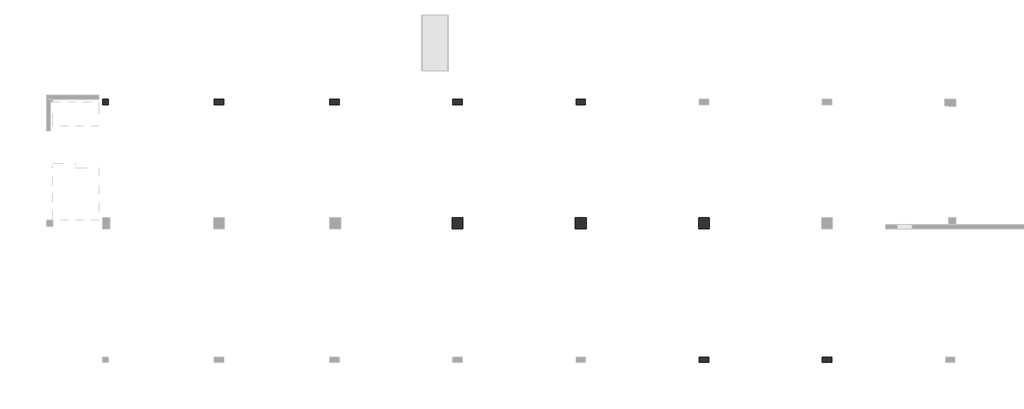
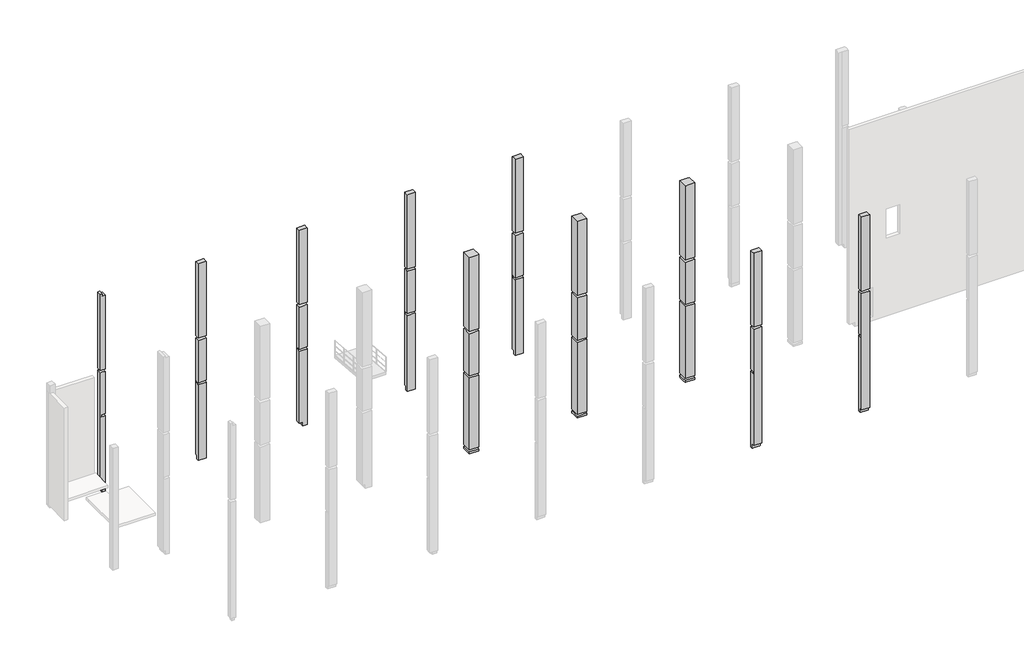
# One storey, part 2 of 3: 10 columns.
"""IFC4 building model written with IfcOpenShell, lengths in millimetres."""

from ifc_helpers import new_model, si_unit, origin, place, context, project, spatial, faceted_brep, element, save

model = new_model("IFC4")

# Units and contexts
model_context = context("Model", 3, world=origin())
ifc_project = project(units=[si_unit("LENGTHUNIT", "METRE", prefix="MILLI")], contexts=[model_context])

# Site, building, storey
site = spatial("IfcSite", under=ifc_project)
building = spatial("IfcBuilding", under=site)
storey = spatial("IfcBuildingStorey", under=building, Name="G.L", Elevation=-150.0381366)

# Columns
placement = place(None, origin())
element("IfcColumn", 1, ObjectType="RC_Column_Rectangular : H_SC_AR_S15_AG_W700xL700_C1", at=placement, inside=storey, context=model_context, shape_type="Brep", body=[
    faceted_brep([(23350.0, 9849.5208589, -150.0381366), (23350.0, 9749.5208589, -150.0381366), (23350.0, 9149.5208589, -150.0381366), (22750.0, 9149.5208589, -150.0381366), (22650.0, 9149.5208589, -150.0381366), (22650.0, 9849.5208589, -150.0381366), (22750.0, 9849.5208589, -150.0381366), (23250.0, 9849.5208589, -150.0381366), (23350.0, 9149.5208589, -0.0381366), (23350.0, 9749.5208589, -0.0381366), (23350.0, 9849.5208589, -0.0381366), (23250.0, 9849.5208589, -0.0381366), (22750.0, 9849.5208589, -0.0381366), (22650.0, 9849.5208589, -0.0381366), (22650.0, 9149.5208589, -0.0381366), (22750.0, 9149.5208589, -0.0381366), (23250.0, 9149.5208589, -0.0381366)], [[[0, 1, 2, 3, 4, 5, 6, 7]], [[8, 9, 10, 11, 12, 13, 14, 15, 16]], [[2, 1, 0, 10, 9, 8]], [[4, 3, 2, 8, 16, 15, 14]], [[5, 4, 14, 13]], [[0, 7, 6, 5, 13, 12, 11, 10]]]),
    faceted_brep([(23350.0, 9149.5208589, 9449.9618634), (23350.0, 9849.5208589, 9449.9618634), (23350.0, 9849.5208589, 15259.9618634), (23350.0, 9724.5208589, 15259.9618634), (23350.0, 9274.5208589, 15259.9618634), (23350.0, 9149.5208589, 15259.9618634), (22650.0, 9149.5208589, 9449.9618634), (23225.0, 9149.5208589, 15259.9618634), (22775.0, 9149.5208589, 15259.9618634), (22650.0, 9149.5208589, 15259.9618634), (22650.0, 9849.5208589, 9449.9618634), (22650.0, 9274.5208589, 15259.9618634), (22650.0, 9724.5208589, 15259.9618634), (22650.0, 9849.5208589, 15259.9618634), (22775.0, 9849.5208589, 15259.9618634), (23225.0, 9849.5208589, 15259.9618634)], [[[0, 1, 2, 3, 4, 5]], [[6, 0, 5, 7, 8, 9]], [[10, 6, 9, 11, 12, 13]], [[1, 10, 13, 14, 15, 2]], [[1, 0, 6, 10]], [[5, 4, 3, 2, 15, 14, 13, 12, 11, 9, 8, 7]]]),
    faceted_brep([(23350.0, 9849.5208589, 149.9618634), (23350.0, 9149.5208589, 149.9618634), (22650.0, 9149.5208589, 149.9618634), (22650.0, 9849.5208589, 149.9618634), (23350.0, 9149.5208589, 5799.9618634), (23350.0, 9199.5208589, 5799.9618634), (23350.0, 9799.5208589, 5799.9618634), (23350.0, 9849.5208589, 5799.9618634), (23250.0, 9849.5208589, 5799.9618634), (22750.0, 9849.5208589, 5799.9618634), (22650.0, 9849.5208589, 5799.9618634), (22650.0, 9799.5208589, 5799.9618634), (22650.0, 9199.5208589, 5799.9618634), (22650.0, 9149.5208589, 5799.9618634), (22750.0, 9149.5208589, 5799.9618634), (23250.0, 9149.5208589, 5799.9618634)], [[[0, 1, 2, 3]], [[4, 5, 6, 7, 8, 9, 10, 11, 12, 13, 14, 15]], [[1, 0, 7, 6, 5, 4]], [[2, 1, 4, 15, 14, 13]], [[3, 2, 13, 12, 11, 10]], [[0, 3, 10, 9, 8, 7]]]),
    faceted_brep([(23350.0, 9849.5208589, 5949.9618634), (23350.0, 9149.5208589, 5949.9618634), (22650.0, 9149.5208589, 5949.9618634), (22650.0, 9849.5208589, 5949.9618634), (23350.0, 9149.5208589, 9269.9618634), (23350.0, 9199.5208589, 9269.9618634), (23350.0, 9799.5208589, 9269.9618634), (23350.0, 9849.5208589, 9269.9618634), (23250.0, 9849.5208589, 9269.9618634), (22750.0, 9849.5208589, 9269.9618634), (22650.0, 9849.5208589, 9269.9618634), (22650.0, 9799.5208589, 9269.9618634), (22650.0, 9199.5208589, 9269.9618634), (22650.0, 9149.5208589, 9269.9618634), (22750.0, 9149.5208589, 9269.9618634), (23250.0, 9149.5208589, 9269.9618634)], [[[0, 1, 2, 3]], [[4, 5, 6, 7, 8, 9, 10, 11, 12, 13, 14, 15]], [[1, 0, 7, 6, 5, 4]], [[2, 1, 4, 15, 14, 13]], [[3, 2, 13, 12, 11, 10]], [[0, 3, 10, 9, 8, 7]]]),
])
element("IfcColumn", 2, ObjectType="RC_Column_Rectangular : H_SC_AR_S15_AG_W700xL700_C1", at=placement, inside=storey, context=model_context, shape_type="Brep", body=[
    faceted_brep([(31350.0, 9849.5208589, -150.0381366), (31350.0, 9749.5208589, -150.0381366), (31350.0, 9149.5208589, -150.0381366), (31250.0, 9149.5208589, -150.0381366), (30650.0, 9149.5208589, -150.0381366), (30650.0, 9749.5208589, -150.0381366), (30650.0, 9849.5208589, -150.0381366), (30750.0, 9849.5208589, -150.0381366), (31250.0, 9849.5208589, -150.0381366), (31350.0, 9149.5208589, -0.0381366), (31350.0, 9749.5208589, -0.0381366), (31350.0, 9849.5208589, -0.0381366), (31250.0, 9849.5208589, -0.0381366), (30750.0, 9849.5208589, -0.0381366), (30650.0, 9849.5208589, -0.0381366), (30650.0, 9749.5208589, -0.0381366), (30650.0, 9149.5208589, -0.0381366), (30750.0, 9149.5208589, -0.0381366), (31250.0, 9149.5208589, -0.0381366)], [[[0, 1, 2, 3, 4, 5, 6, 7, 8]], [[9, 10, 11, 12, 13, 14, 15, 16, 17, 18]], [[2, 1, 0, 11, 10, 9]], [[4, 3, 2, 9, 18, 17, 16]], [[6, 5, 4, 16, 15, 14]], [[0, 8, 7, 6, 14, 13, 12, 11]]]),
    faceted_brep([(31350.0, 9149.5208589, 9449.9618634), (31350.0, 9849.5208589, 9449.9618634), (31350.0, 9849.5208589, 15259.9618634), (31350.0, 9724.5208589, 15259.9618634), (31350.0, 9274.5208589, 15259.9618634), (31350.0, 9149.5208589, 15259.9618634), (30650.0, 9149.5208589, 9449.9618634), (31225.0, 9149.5208589, 15259.9618634), (30775.0, 9149.5208589, 15259.9618634), (30650.0, 9149.5208589, 15259.9618634), (30650.0, 9849.5208589, 9449.9618634), (30650.0, 9274.5208589, 15259.9618634), (30650.0, 9724.5208589, 15259.9618634), (30650.0, 9849.5208589, 15259.9618634), (30775.0, 9849.5208589, 15259.9618634), (31225.0, 9849.5208589, 15259.9618634)], [[[0, 1, 2, 3, 4, 5]], [[6, 0, 5, 7, 8, 9]], [[10, 6, 9, 11, 12, 13]], [[1, 10, 13, 14, 15, 2]], [[1, 0, 6, 10]], [[5, 4, 3, 2, 15, 14, 13, 12, 11, 9, 8, 7]]]),
    faceted_brep([(31350.0, 9849.5208589, 149.9618634), (31350.0, 9149.5208589, 149.9618634), (30650.0, 9149.5208589, 149.9618634), (30650.0, 9849.5208589, 149.9618634), (31350.0, 9149.5208589, 5799.9618634), (31350.0, 9199.5208589, 5799.9618634), (31350.0, 9799.5208589, 5799.9618634), (31350.0, 9849.5208589, 5799.9618634), (31250.0, 9849.5208589, 5799.9618634), (30750.0, 9849.5208589, 5799.9618634), (30650.0, 9849.5208589, 5799.9618634), (30650.0, 9799.5208589, 5799.9618634), (30650.0, 9199.5208589, 5799.9618634), (30650.0, 9149.5208589, 5799.9618634), (30750.0, 9149.5208589, 5799.9618634), (31250.0, 9149.5208589, 5799.9618634)], [[[0, 1, 2, 3]], [[4, 5, 6, 7, 8, 9, 10, 11, 12, 13, 14, 15]], [[1, 0, 7, 6, 5, 4]], [[2, 1, 4, 15, 14, 13]], [[3, 2, 13, 12, 11, 10]], [[0, 3, 10, 9, 8, 7]]]),
    faceted_brep([(31350.0, 9849.5208589, 5949.9618634), (31350.0, 9149.5208589, 5949.9618634), (30650.0, 9149.5208589, 5949.9618634), (30650.0, 9849.5208589, 5949.9618634), (31350.0, 9149.5208589, 9269.9618634), (31350.0, 9199.5208589, 9269.9618634), (31350.0, 9799.5208589, 9269.9618634), (31350.0, 9849.5208589, 9269.9618634), (31250.0, 9849.5208589, 9269.9618634), (30750.0, 9849.5208589, 9269.9618634), (30650.0, 9849.5208589, 9269.9618634), (30650.0, 9799.5208589, 9269.9618634), (30650.0, 9199.5208589, 9269.9618634), (30650.0, 9149.5208589, 9269.9618634), (30750.0, 9149.5208589, 9269.9618634), (31250.0, 9149.5208589, 9269.9618634)], [[[0, 1, 2, 3]], [[4, 5, 6, 7, 8, 9, 10, 11, 12, 13, 14, 15]], [[1, 0, 7, 6, 5, 4]], [[2, 1, 4, 15, 14, 13]], [[3, 2, 13, 12, 11, 10]], [[0, 3, 10, 9, 8, 7]]]),
])
element("IfcColumn", 3, ObjectType="RC_Column_Rectangular : H_SC_AR_S15_AG_W700xL700_C1", at=placement, inside=storey, context=model_context, shape_type="Brep", body=[
    faceted_brep([(39350.0, 9849.5208589, -150.0381366), (39350.0, 9749.5208589, -150.0381366), (39350.0, 9149.5208589, -150.0381366), (38750.0, 9149.5208589, -150.0381366), (38749.6109568, 9149.5208589, -150.0381366), (38650.0, 9149.5208589, -150.0381366), (38650.0, 9499.9097478, -150.0381366), (38650.0, 9749.5208589, -150.0381366), (38650.0, 9849.5208589, -150.0381366), (38750.0, 9849.5208589, -150.0381366), (39250.0, 9849.5208589, -150.0381366), (39350.0, 9149.5208589, -0.0381366), (39350.0, 9749.5208589, -0.0381366), (39350.0, 9849.5208589, -0.0381366), (39250.0, 9849.5208589, -0.0381366), (38750.0, 9849.5208589, -0.0381366), (38650.0, 9849.5208589, -0.0381366), (38650.0, 9749.5208589, -0.0381366), (38650.0, 9499.9097478, -0.0381366), (38650.0, 9149.5208589, -0.0381366)], [[[0, 1, 2, 3, 4, 5, 6, 7, 8, 9, 10]], [[11, 12, 13, 14, 15, 16, 17, 18, 19]], [[2, 1, 0, 13, 12, 11]], [[5, 4, 3, 2, 11, 19]], [[8, 7, 6, 5, 19, 18, 17, 16]], [[0, 10, 9, 8, 16, 15, 14, 13]]]),
    faceted_brep([(39350.0, 9149.5208589, 9449.9618634), (39350.0, 9849.5208589, 9449.9618634), (39350.0, 9849.5208589, 15259.9618634), (39350.0, 9149.5208589, 15259.9618634), (38650.0, 9149.5208589, 9449.9618634), (38650.0, 9149.5208589, 15259.9618634), (38650.0, 9849.5208589, 9449.9618634), (38650.0, 9849.5208589, 15259.9618634), (38775.0, 9849.5208589, 15259.9618634), (39225.0, 9849.5208589, 15259.9618634)], [[[0, 1, 2, 3]], [[4, 0, 3, 5]], [[6, 4, 5, 7]], [[1, 6, 7, 8, 9, 2]], [[1, 0, 4, 6]], [[3, 2, 9, 8, 7, 5]]]),
    faceted_brep([(39350.0, 9849.5208589, 149.9618634), (39350.0, 9149.5208589, 149.9618634), (38650.0, 9149.5208589, 149.9618634), (38650.0, 9849.5208589, 149.9618634), (39350.0, 9149.5208589, 5799.9618634), (39350.0, 9199.5208589, 5799.9618634), (39350.0, 9799.5208589, 5799.9618634), (39350.0, 9849.5208589, 5799.9618634), (39250.0, 9849.5208589, 5799.9618634), (38750.0, 9849.5208589, 5799.9618634), (38650.0, 9849.5208589, 5799.9618634), (38650.0, 9799.5208589, 5799.9618634), (38650.0, 9199.5208589, 5799.9618634), (38650.0, 9149.5208589, 5799.9618634)], [[[0, 1, 2, 3]], [[4, 5, 6, 7, 8, 9, 10, 11, 12, 13]], [[1, 0, 7, 6, 5, 4]], [[2, 1, 4, 13]], [[3, 2, 13, 12, 11, 10]], [[0, 3, 10, 9, 8, 7]]]),
    faceted_brep([(39350.0, 9849.5208589, 5949.9618634), (39350.0, 9149.5208589, 5949.9618634), (38650.0, 9149.5208589, 5949.9618634), (38650.0, 9849.5208589, 5949.9618634), (39350.0, 9149.5208589, 9269.9618634), (39350.0, 9199.5208589, 9269.9618634), (39350.0, 9799.5208589, 9269.9618634), (39350.0, 9849.5208589, 9269.9618634), (39250.0, 9849.5208589, 9269.9618634), (38750.0, 9849.5208589, 9269.9618634), (38650.0, 9849.5208589, 9269.9618634), (38650.0, 9799.5208589, 9269.9618634), (38650.0, 9199.5208589, 9269.9618634), (38650.0, 9149.5208589, 9269.9618634)], [[[0, 1, 2, 3]], [[4, 5, 6, 7, 8, 9, 10, 11, 12, 13]], [[1, 0, 7, 6, 5, 4]], [[2, 1, 4, 13]], [[3, 2, 13, 12, 11, 10]], [[0, 3, 10, 9, 8, 7]]]),
])
element("IfcColumn", 4, ObjectType="RC_Column_Rectangular : H_SC_AR_S15_AG_W600xL600_C2", at=placement, inside=storey, context=model_context, shape_type="Brep", body=[
    faceted_brep([(300.0, 17199.5208589, -150.0381366), (100.0, 17199.5208589, -150.0381366), (100.0, 17399.5208589, -150.0381366), (300.0, 17399.5208589, -150.0381366), (300.0, 17499.5208589, 5799.9618634), (0.0, 17499.5208589, 5799.9618634), (0.0, 17199.5208589, 5799.9618634), (100.0, 17199.5208589, 5799.9618634), (150.0, 17199.5208589, 5799.9618634), (300.0, 17199.5208589, 5799.9618634), (300.0, 17399.5208589, 5799.9618634), (0.0, 17199.5208589, 5949.9618634), (0.0, 17499.5208589, 5949.9618634), (300.0, 17499.5208589, 5949.9618634), (300.0, 17199.5208589, 5949.9618634), (0.0, 17199.5208589, 5899.9618634), (300.0, 17199.5208589, 9269.9618634), (300.0, 17399.5208589, 9269.9618634), (300.0, 17549.5208589, 9269.9618634), (-50.0, 17549.5208589, 9269.9618634), (-50.0, 17199.5208589, 9269.9618634), (100.0, 17199.5208589, 9269.9618634), (100.0, 17199.5208589, 149.9618634), (100.0, 17399.5208589, 149.9618634), (-50.0, 17199.5208589, 149.9618634), (-50.0, 17549.5208589, 149.9618634), (300.0, 17549.5208589, 149.9618634), (300.0, 17399.5208589, 149.9618634), (300.0, 17549.5208589, 8749.9618634), (300.0, 17549.5208589, 5949.9618634), (300.0, 17549.5208589, 5249.9618634), (-50.0, 17199.5208589, 8749.9618634), (-50.0, 17199.5208589, 5949.9618634), (-50.0, 17199.5208589, 5899.9618634), (-50.0, 17199.5208589, 5199.9618634)], [[[0, 1, 2, 3]], [[4, 5, 6, 7, 8, 9, 10]], [[11, 12, 13, 14]], [[5, 12, 11, 15, 6]], [[12, 5, 4, 13]], [[16, 17, 18, 19, 20, 21]], [[22, 23, 2, 1]], [[23, 22, 24, 25, 26, 27]], [[18, 28, 29, 30, 26, 25, 19]], [[9, 0, 3, 27, 26, 30, 29, 28, 18, 17, 16, 14, 13, 4, 10]], [[0, 9, 8, 7, 6, 15, 11, 14, 16, 21, 20, 31, 32, 33, 34, 24, 22, 1]], [[25, 24, 34, 33, 32, 31, 20, 19]], [[23, 27, 3, 2]]]),
    faceted_brep([(300.0, 17199.5208589, 9449.9618634), (300.0, 17549.5208589, 9449.9618634), (300.0, 17549.5208589, 14709.9618634), (300.0, 17549.5208589, 15259.9618634), (300.0, 17399.5208589, 15259.9618634), (300.0, 17199.5208589, 15259.9618634), (-50.0, 17199.5208589, 9449.9618634), (100.0, 17199.5208589, 15259.9618634), (100.0, 17199.5208589, 15409.9618634), (-50.0, 17199.5208589, 15409.9618634), (-50.0, 17199.5208589, 14709.9618634), (100.0, 17549.5208589, 15409.9618634), (-50.0, 17549.5208589, 15409.9618634), (-50.0, 17549.5208589, 9449.9618634), (100.0, 17549.5208589, 15259.9618634)], [[[0, 1, 2, 3, 4, 5]], [[6, 0, 5, 7, 8, 9, 10]], [[8, 11, 12, 9]], [[1, 0, 6, 13]], [[14, 7, 5, 4, 3]], [[7, 14, 11, 8]], [[6, 10, 9, 12, 13]], [[3, 2, 1, 13, 12, 11, 14]]]),
])
element("IfcColumn", 5, ObjectType="RC_Column_Rectangular : H_SC_AR_S15_AG_W600xL600_C2", at=placement, inside=storey, context=model_context, shape_type="Brep", body=[
    faceted_brep([(7800.0, 17199.5208589, -150.0381366), (7200.0, 17199.5208589, -150.0381366), (7200.0, 17399.5208589, -150.0381366), (7800.0, 17399.5208589, -150.0381366), (7800.0, 17499.5208589, 5799.9618634), (7200.0, 17499.5208589, 5799.9618634), (7200.0, 17399.5208589, 5799.9618634), (7200.0, 17199.5208589, 5799.9618634), (7250.0, 17199.5208589, 5799.9618634), (7750.0, 17199.5208589, 5799.9618634), (7800.0, 17199.5208589, 5799.9618634), (7800.0, 17399.5208589, 5799.9618634), (7200.0, 17499.5208589, 5949.9618634), (7800.0, 17499.5208589, 5949.9618634), (7800.0, 17199.5208589, 5949.9618634), (7200.0, 17199.5208589, 5949.9618634), (7800.0, 17199.5208589, 9269.9618634), (7800.0, 17399.5208589, 9269.9618634), (7800.0, 17549.5208589, 9269.9618634), (7200.0, 17549.5208589, 9269.9618634), (7200.0, 17399.5208589, 9269.9618634), (7200.0, 17199.5208589, 9269.9618634), (7250.0, 17199.5208589, 9269.9618634), (7750.0, 17199.5208589, 9269.9618634), (7800.0, 17549.5208589, 8749.9618634), (7800.0, 17549.5208589, 5949.9618634), (7800.0, 17549.5208589, 5249.9618634), (7800.0, 17549.5208589, 149.9618634), (7200.0, 17549.5208589, 149.9618634), (7200.0, 17549.5208589, 5249.9618634), (7200.0, 17549.5208589, 5949.9618634), (7200.0, 17549.5208589, 8749.9618634), (7800.0, 17399.5208589, 149.9618634), (7200.0, 17399.5208589, 149.9618634)], [[[0, 1, 2, 3]], [[4, 5, 6, 7, 8, 9, 10, 11]], [[12, 13, 14, 15]], [[5, 4, 13, 12]], [[1, 0, 10, 9, 8, 7]], [[16, 17, 18, 19, 20, 21, 22, 23]], [[15, 14, 16, 23, 22, 21]], [[18, 24, 25, 26, 27, 28, 29, 30, 31, 19]], [[10, 0, 3, 32, 27, 26, 25, 24, 18, 17, 16, 14, 13, 4, 11]], [[1, 7, 6, 5, 12, 15, 21, 20, 19, 31, 30, 29, 28, 33, 2]], [[33, 32, 3, 2]], [[32, 33, 28, 27]]]),
    faceted_brep([(7800.0, 17199.5208589, 9449.9618634), (7800.0, 17549.5208589, 9449.9618634), (7800.0, 17549.5208589, 14709.9618634), (7800.0, 17549.5208589, 15259.9618634), (7800.0, 17399.5208589, 15259.9618634), (7800.0, 17199.5208589, 15259.9618634), (7200.0, 17199.5208589, 9449.9618634), (7725.0, 17199.5208589, 15259.9618634), (7275.0, 17199.5208589, 15259.9618634), (7200.0, 17199.5208589, 15259.9618634), (7200.0, 17549.5208589, 9449.9618634), (7200.0, 17399.5208589, 15259.9618634), (7200.0, 17549.5208589, 15259.9618634), (7200.0, 17549.5208589, 14709.9618634)], [[[0, 1, 2, 3, 4, 5]], [[6, 0, 5, 7, 8, 9]], [[10, 6, 9, 11, 12, 13]], [[1, 0, 6, 10]], [[5, 4, 3, 12, 11, 9, 8, 7]], [[3, 2, 1, 10, 13, 12]]]),
])
element("IfcColumn", 6, ObjectType="RC_Column_Rectangular : H_SC_AR_S15_AG_W600xL600_C2", at=placement, inside=storey, context=model_context, shape_type="Brep", body=[
    faceted_brep([(15300.0, 17199.5208589, -150.0381366), (14950.0, 17199.5208589, -150.0381366), (14950.0, 17399.5208589, -150.0381366), (15300.0, 17399.5208589, -150.0381366), (15300.0, 17499.5208589, 5799.9618634), (14700.0, 17499.5208589, 5799.9618634), (14700.0, 17399.5208589, 5799.9618634), (14700.0, 17199.5208589, 5799.9618634), (14750.0, 17199.5208589, 5799.9618634), (15250.0, 17199.5208589, 5799.9618634), (15300.0, 17199.5208589, 5799.9618634), (15300.0, 17399.5208589, 5799.9618634), (14700.0, 17499.5208589, 5949.9618634), (15300.0, 17499.5208589, 5949.9618634), (15300.0, 17199.5208589, 5949.9618634), (14700.0, 17199.5208589, 5949.9618634), (15300.0, 17199.5208589, -0.0381366), (15300.0, 17199.5208589, 149.9618634), (14700.0, 17199.5208589, 149.9618634), (14950.0, 17199.5208589, 149.9618634), (14950.0, 17199.5208589, -0.0381366), (15300.0, 17199.5208589, 9269.9618634), (15300.0, 17399.5208589, 9269.9618634), (15300.0, 17549.5208589, 9269.9618634), (14700.0, 17549.5208589, 9269.9618634), (14700.0, 17399.5208589, 9269.9618634), (14700.0, 17199.5208589, 9269.9618634), (14750.0, 17199.5208589, 9269.9618634), (15250.0, 17199.5208589, 9269.9618634), (14700.0, 17549.5208589, 149.9618634), (14700.0, 17549.5208589, 5249.9618634), (14700.0, 17549.5208589, 5949.9618634), (14700.0, 17549.5208589, 8749.9618634), (15300.0, 17549.5208589, 8749.9618634), (15300.0, 17549.5208589, 5949.9618634), (15300.0, 17549.5208589, 5249.9618634), (15300.0, 17549.5208589, 149.9618634), (14700.0, 17399.5208589, 149.9618634), (14950.0, 17399.5208589, 149.9618634), (15300.0, 17399.5208589, 149.9618634), (15300.0, 17399.5208589, -0.0381366)], [[[0, 1, 2, 3]], [[4, 5, 6, 7, 8, 9, 10, 11]], [[12, 13, 14, 15]], [[5, 4, 13, 12]], [[0, 16, 17, 10, 9, 8, 7, 18, 19, 20, 1]], [[21, 22, 23, 24, 25, 26, 27, 28]], [[15, 14, 21, 28, 27, 26]], [[29, 30, 31, 32, 24, 23, 33, 34, 35, 36]], [[7, 6, 5, 12, 15, 26, 25, 24, 32, 31, 30, 29, 37, 18]], [[19, 38, 2, 1, 20]], [[38, 19, 18, 37, 29, 36, 39]], [[16, 0, 3, 40, 39, 36, 35, 34, 33, 23, 22, 21, 14, 13, 4, 11, 10, 17]], [[38, 39, 40, 3, 2]]]),
    faceted_brep([(15300.0, 17199.5208589, 9449.9618634), (15300.0, 17549.5208589, 9449.9618634), (15300.0, 17549.5208589, 14709.9618634), (15300.0, 17549.5208589, 15259.9618634), (15300.0, 17399.5208589, 15259.9618634), (15300.0, 17199.5208589, 15259.9618634), (14700.0, 17199.5208589, 9449.9618634), (15225.0, 17199.5208589, 15259.9618634), (14775.0, 17199.5208589, 15259.9618634), (14700.0, 17199.5208589, 15259.9618634), (14700.0, 17549.5208589, 9449.9618634), (14700.0, 17399.5208589, 15259.9618634), (14700.0, 17549.5208589, 15259.9618634), (14700.0, 17549.5208589, 14709.9618634)], [[[0, 1, 2, 3, 4, 5]], [[6, 0, 5, 7, 8, 9]], [[10, 6, 9, 11, 12, 13]], [[1, 0, 6, 10]], [[5, 4, 3, 12, 11, 9, 8, 7]], [[10, 13, 12, 3, 2, 1]]]),
])
element("IfcColumn", 7, ObjectType="RC_Column_Rectangular : H_SC_AR_S15_AG_W600xL600_C2", at=placement, inside=storey, context=model_context, shape_type="Brep", body=[
    faceted_brep([(23300.0, 17199.5208589, -150.0381366), (22700.0, 17199.5208589, -150.0381366), (22700.0, 17399.5208589, -150.0381366), (23300.0, 17399.5208589, -150.0381366), (23300.0, 17499.5208589, 5799.9618634), (22700.0, 17499.5208589, 5799.9618634), (22700.0, 17399.5208589, 5799.9618634), (22700.0, 17199.5208589, 5799.9618634), (22750.0, 17199.5208589, 5799.9618634), (23250.0, 17199.5208589, 5799.9618634), (23300.0, 17199.5208589, 5799.9618634), (23300.0, 17399.5208589, 5799.9618634), (22700.0, 17499.5208589, 5949.9618634), (23300.0, 17499.5208589, 5949.9618634), (23300.0, 17199.5208589, 5949.9618634), (22700.0, 17199.5208589, 5949.9618634), (23300.0, 17199.5208589, -0.0381366), (23300.0, 17199.5208589, 149.9618634), (22700.0, 17199.5208589, 149.9618634), (22700.0, 17199.5208589, -0.0381366), (23300.0, 17199.5208589, 9269.9618634), (23300.0, 17399.5208589, 9269.9618634), (23300.0, 17549.5208589, 9269.9618634), (22700.0, 17549.5208589, 9269.9618634), (22700.0, 17399.5208589, 9269.9618634), (22700.0, 17199.5208589, 9269.9618634), (22750.0, 17199.5208589, 9269.9618634), (23250.0, 17199.5208589, 9269.9618634), (22700.0, 17549.5208589, 149.9618634), (22700.0, 17549.5208589, 5249.9618634), (22700.0, 17549.5208589, 5949.9618634), (22700.0, 17549.5208589, 8749.9618634), (23300.0, 17549.5208589, 8749.9618634), (23300.0, 17549.5208589, 5949.9618634), (23300.0, 17549.5208589, 5249.9618634), (23300.0, 17549.5208589, 149.9618634), (22700.0, 17399.5208589, 149.9618634), (22700.0, 17399.5208589, -0.0381366), (23300.0, 17399.5208589, -0.0381366), (23300.0, 17399.5208589, 149.9618634)], [[[0, 1, 2, 3]], [[4, 5, 6, 7, 8, 9, 10, 11]], [[12, 13, 14, 15]], [[5, 4, 13, 12]], [[1, 0, 16, 17, 10, 9, 8, 7, 18, 19]], [[20, 21, 22, 23, 24, 25, 26, 27]], [[15, 14, 20, 27, 26, 25]], [[28, 29, 30, 31, 23, 22, 32, 33, 34, 35]], [[1, 19, 18, 7, 6, 5, 12, 15, 25, 24, 23, 31, 30, 29, 28, 36, 37, 2]], [[16, 0, 3, 38, 39, 35, 34, 33, 32, 22, 21, 20, 14, 13, 4, 11, 10, 17]], [[36, 39, 38, 3, 2, 37]], [[39, 36, 28, 35]]]),
    faceted_brep([(23300.0, 17199.5208589, 9449.9618634), (23300.0, 17549.5208589, 9449.9618634), (23300.0, 17549.5208589, 14709.9618634), (23300.0, 17549.5208589, 15259.9618634), (23300.0, 17399.5208589, 15259.9618634), (23300.0, 17199.5208589, 15259.9618634), (22700.0, 17199.5208589, 9449.9618634), (23225.0, 17199.5208589, 15259.9618634), (22775.0, 17199.5208589, 15259.9618634), (22700.0, 17199.5208589, 15259.9618634), (22700.0, 17549.5208589, 9449.9618634), (22700.0, 17399.5208589, 15259.9618634), (22700.0, 17549.5208589, 15259.9618634), (22700.0, 17549.5208589, 14709.9618634)], [[[0, 1, 2, 3, 4, 5]], [[6, 0, 5, 7, 8, 9]], [[10, 6, 9, 11, 12, 13]], [[1, 0, 6, 10]], [[5, 4, 3, 12, 11, 9, 8, 7]], [[10, 13, 12, 3, 2, 1]]]),
])
element("IfcColumn", 8, ObjectType="RC_Column_Rectangular : H_SC_AR_S15_AG_W600xL600_C2", at=placement, inside=storey, context=model_context, shape_type="Brep", body=[
    faceted_brep([(31300.0, 17199.5208589, -150.0381366), (30700.0, 17199.5208589, -150.0381366), (30700.0, 17399.5208589, -150.0381366), (31300.0, 17399.5208589, -150.0381366), (31300.0, 17499.5208589, 5799.9618634), (30700.0, 17499.5208589, 5799.9618634), (30700.0, 17399.5208589, 5799.9618634), (30700.0, 17199.5208589, 5799.9618634), (30750.0, 17199.5208589, 5799.9618634), (31250.0, 17199.5208589, 5799.9618634), (31300.0, 17199.5208589, 5799.9618634), (31300.0, 17399.5208589, 5799.9618634), (30700.0, 17499.5208589, 5949.9618634), (31300.0, 17499.5208589, 5949.9618634), (31300.0, 17199.5208589, 5949.9618634), (30700.0, 17199.5208589, 5949.9618634), (31300.0, 17199.5208589, -0.0381366), (31300.0, 17199.5208589, 149.9618634), (30700.0, 17199.5208589, 149.9618634), (30700.0, 17199.5208589, -0.0381366), (31300.0, 17199.5208589, 9269.9618634), (31300.0, 17399.5208589, 9269.9618634), (31300.0, 17549.5208589, 9269.9618634), (30700.0, 17549.5208589, 9269.9618634), (30700.0, 17399.5208589, 9269.9618634), (30700.0, 17199.5208589, 9269.9618634), (30750.0, 17199.5208589, 9269.9618634), (31250.0, 17199.5208589, 9269.9618634), (30700.0, 17549.5208589, 149.9618634), (30700.0, 17549.5208589, 5249.9618634), (30700.0, 17549.5208589, 5949.9618634), (30700.0, 17549.5208589, 8749.9618634), (31300.0, 17549.5208589, 8749.9618634), (31300.0, 17549.5208589, 5949.9618634), (31300.0, 17549.5208589, 5249.9618634), (31300.0, 17549.5208589, 149.9618634), (30700.0, 17399.5208589, 149.9618634), (30700.0, 17399.5208589, -0.0381366), (31300.0, 17399.5208589, -0.0381366), (31300.0, 17399.5208589, 149.9618634)], [[[0, 1, 2, 3]], [[4, 5, 6, 7, 8, 9, 10, 11]], [[12, 13, 14, 15]], [[5, 4, 13, 12]], [[1, 0, 16, 17, 10, 9, 8, 7, 18, 19]], [[20, 21, 22, 23, 24, 25, 26, 27]], [[15, 14, 20, 27, 26, 25]], [[28, 29, 30, 31, 23, 22, 32, 33, 34, 35]], [[1, 19, 18, 7, 6, 5, 12, 15, 25, 24, 23, 31, 30, 29, 28, 36, 37, 2]], [[16, 0, 3, 38, 39, 35, 34, 33, 32, 22, 21, 20, 14, 13, 4, 11, 10, 17]], [[36, 39, 38, 3, 2, 37]], [[39, 36, 28, 35]]]),
    faceted_brep([(31300.0, 17199.5208589, 9449.9618634), (31300.0, 17549.5208589, 9449.9618634), (31300.0, 17549.5208589, 14709.9618634), (31300.0, 17549.5208589, 15259.9618634), (31300.0, 17399.5208589, 15259.9618634), (31300.0, 17199.5208589, 15259.9618634), (30700.0, 17199.5208589, 9449.9618634), (31225.0, 17199.5208589, 15259.9618634), (30775.0, 17199.5208589, 15259.9618634), (30700.0, 17199.5208589, 15259.9618634), (30700.0, 17549.5208589, 9449.9618634), (30700.0, 17399.5208589, 15259.9618634), (30700.0, 17549.5208589, 15259.9618634), (30700.0, 17549.5208589, 14709.9618634)], [[[0, 1, 2, 3, 4, 5]], [[6, 0, 5, 7, 8, 9]], [[10, 6, 9, 11, 12, 13]], [[1, 0, 6, 10]], [[5, 4, 3, 12, 11, 9, 8, 7]], [[10, 13, 12, 3, 2, 1]]]),
])
element("IfcColumn", 9, ObjectType="RC_Column_Rectangular : H_SC_AR_S15_AG_W600xL600_C2", at=placement, inside=storey, context=model_context, shape_type="Brep", body=[
    faceted_brep([(46700.0, 799.5208589, -150.0381366), (47300.0, 799.5208589, -150.0381366), (47300.0, 599.5208589, -150.0381366), (46700.0, 599.5208589, -150.0381366), (46700.0, 499.5208589, 5799.9618634), (47300.0, 499.5208589, 5799.9618634), (47300.0, 599.5208589, 5799.9618634), (47300.0, 799.5208589, 5799.9618634), (47250.0, 799.5208589, 5799.9618634), (46750.0, 799.5208589, 5799.9618634), (46700.0, 799.5208589, 5799.9618634), (46700.0, 599.5208589, 5799.9618634), (47300.0, 499.5208589, 5949.9618634), (46700.0, 499.5208589, 5949.9618634), (46700.0, 799.5208589, 5949.9618634), (47300.0, 799.5208589, 5949.9618634), (46700.0, 799.5208589, -0.0381366), (46700.0, 799.5208589, 149.9618634), (47300.0, 799.5208589, 149.9618634), (47300.0, 799.5208589, -0.0381366), (47300.0, 449.5208589, 9269.9618634), (47300.0, 599.5208589, 9269.9618634), (47300.0, 799.5208589, 9269.9618634), (47250.0, 799.5208589, 9269.9618634), (46750.0, 799.5208589, 9269.9618634), (46700.0, 799.5208589, 9269.9618634), (46700.0, 599.5208589, 9269.9618634), (46700.0, 449.5208589, 9269.9618634), (47300.0, 599.5208589, 149.9618634), (46700.0, 599.5208589, 149.9618634), (47300.0, 449.5208589, 149.9618634), (46700.0, 449.5208589, 149.9618634), (47300.0, 449.5208589, 5249.9618634), (47300.0, 449.5208589, 5949.9618634), (47300.0, 449.5208589, 8749.9618634), (46700.0, 449.5208589, 8749.9618634), (46700.0, 449.5208589, 5949.9618634), (46700.0, 449.5208589, 5249.9618634)], [[[0, 1, 2, 3]], [[4, 5, 6, 7, 8, 9, 10, 11]], [[12, 13, 14, 15]], [[5, 4, 13, 12]], [[1, 0, 16, 17, 10, 9, 8, 7, 18, 19]], [[20, 21, 22, 23, 24, 25, 26, 27]], [[15, 14, 25, 24, 23, 22]], [[28, 29, 3, 2]], [[29, 28, 30, 31]], [[30, 32, 33, 34, 20, 27, 35, 36, 37, 31]], [[1, 19, 18, 7, 6, 5, 12, 15, 22, 21, 20, 34, 33, 32, 30, 28, 2]], [[16, 0, 3, 29, 31, 37, 36, 35, 27, 26, 25, 14, 13, 4, 11, 10, 17]]]),
    faceted_brep([(47300.0, 449.5208589, 9449.9618634), (47300.0, 799.5208589, 9449.9618634), (47300.0, 799.5208589, 15259.9618634), (47300.0, 599.5208589, 15259.9618634), (47300.0, 449.5208589, 15259.9618634), (47300.0, 449.5208589, 14709.9618634), (46700.0, 799.5208589, 9449.9618634), (46700.0, 449.5208589, 9449.9618634), (46700.0, 449.5208589, 14709.9618634), (46700.0, 449.5208589, 15259.9618634), (46700.0, 599.5208589, 15259.9618634), (46700.0, 799.5208589, 15259.9618634), (46775.0, 799.5208589, 15259.9618634), (47225.0, 799.5208589, 15259.9618634)], [[[0, 1, 2, 3, 4, 5]], [[6, 7, 8, 9, 10, 11]], [[1, 6, 11, 12, 13, 2]], [[1, 0, 7, 6]], [[4, 3, 2, 13, 12, 11, 10, 9]], [[0, 5, 4, 9, 8, 7]]]),
])
element("IfcColumn", 10, ObjectType="RC_Column_Rectangular : H_SC_AR_S15_AG_W600xL600_C2", at=placement, inside=storey, context=model_context, shape_type="Brep", body=[
    faceted_brep([(38700.0, 799.5208589, -150.0381366), (38850.0, 799.5208589, -150.0381366), (39240.3334877, 799.5208589, -150.0381366), (39300.0, 799.5208589, -150.0381366), (39300.0, 599.5208589, -150.0381366), (39240.1112654, 599.5208589, -150.0381366), (38850.0, 599.5208589, -150.0381366), (38700.0, 599.5208589, -150.0381366), (38700.0, 499.5208589, 5799.9618634), (39300.0, 499.5208589, 5799.9618634), (39300.0, 599.5208589, 5799.9618634), (39300.0, 799.5208589, 5799.9618634), (39240.3469879, 799.5208589, 5799.9618634), (38740.3466537, 799.5208589, 5799.9618634), (38700.0, 799.5208589, 5799.9618634), (38700.0, 599.5208589, 5799.9618634), (39300.0, 499.5208589, 5949.9618634), (38700.0, 499.5208589, 5949.9618634), (38700.0, 799.5208589, 5949.9618634), (39300.0, 799.5208589, 5949.9618634), (38700.0, 799.5208589, -0.0381366), (38700.0, 799.5208589, 149.9618634), (39300.0, 799.5208589, 149.9618634), (39300.0, 799.5208589, -0.0381366), (39300.0, 449.5208589, 9269.9618634), (39300.0, 599.5208589, 9269.9618634), (39300.0, 799.5208589, 9269.9618634), (39240.3469879, 799.5208589, 9269.9618634), (38740.3466537, 799.5208589, 9269.9618634), (38700.0, 799.5208589, 9269.9618634), (38700.0, 599.5208589, 9269.9618634), (38700.0, 449.5208589, 9269.9618634), (39300.0, 599.5208589, 149.9618634), (38700.0, 599.5208589, 149.9618634), (39300.0, 449.5208589, 149.9618634), (38700.0, 449.5208589, 149.9618634), (39300.0, 449.5208589, 5249.9618634), (39300.0, 449.5208589, 5949.9618634), (39300.0, 449.5208589, 8749.9618634), (38700.0, 449.5208589, 8749.9618634), (38700.0, 449.5208589, 5949.9618634), (38700.0, 449.5208589, 5249.9618634)], [[[0, 1, 2, 3, 4, 5, 6, 7]], [[8, 9, 10, 11, 12, 13, 14, 15]], [[16, 17, 18, 19]], [[9, 8, 17, 16]], [[3, 2, 1, 0, 20, 21, 14, 13, 12, 11, 22, 23]], [[24, 25, 26, 27, 28, 29, 30, 31]], [[19, 18, 29, 28, 27, 26]], [[7, 6, 5, 4, 32, 33]], [[33, 32, 34, 35]], [[34, 36, 37, 38, 24, 31, 39, 40, 41, 35]], [[11, 10, 9, 16, 19, 26, 25, 24, 38, 37, 36, 34, 32, 4, 3, 23, 22]], [[20, 0, 7, 33, 35, 41, 40, 39, 31, 30, 29, 18, 17, 8, 15, 14, 21]]]),
    faceted_brep([(39300.0, 449.5208589, 9449.9618634), (39300.0, 799.5208589, 9449.9618634), (39300.0, 799.5208589, 15259.9618634), (39300.0, 599.5208589, 15259.9618634), (39300.0, 449.5208589, 15259.9618634), (39300.0, 449.5208589, 14709.9618634), (38700.0, 799.5208589, 9449.9618634), (38700.0, 449.5208589, 9449.9618634), (38700.0, 449.5208589, 14709.9618634), (38700.0, 449.5208589, 15259.9618634), (38700.0, 599.5208589, 15259.9618634), (38700.0, 799.5208589, 15259.9618634), (38765.3466705, 799.5208589, 15259.9618634), (39215.3469712, 799.5208589, 15259.9618634)], [[[0, 1, 2, 3, 4, 5]], [[6, 7, 8, 9, 10, 11]], [[1, 6, 11, 12, 13, 2]], [[1, 0, 7, 6]], [[4, 3, 2, 13, 12, 11, 10, 9]], [[0, 5, 4, 9, 8, 7]]]),
])

save(model, "model.ifc")

# Revit data of these elements
# Type "RC_Column_Rectangular : H_SC_AR_S15_AG_W700xL700_C1"
#   Type Comments = "CV-AG"
#   Type Mark = "C1"
#   H_Q'ty Cal Type Tag = "SB-Q1A"
#   H_WM Code_1 = "A03AF032-00022 |  | M3 | Concrete Work | Superstructure Work | Structural Concrete | Cement Type-1 | 25MPa ≤ F'c (Cylinder Strength) < 30MPa |  |  |  |  | A03AF032-00022 Concrete Work Superstructure Work Structural Concrete  Cement Type-1 25MPa ≤ F'c (Cylinder Strength) < 30MPa      |  F'c (Cylinder Strength) = 24MPa"
#   H_WM Code_2 = "A03AD037-00002 |  | TON | Concrete Work | Substructure Work | Rebar Work | Deformed Bar (Non-Coat.) | 400MPa<Fy≤470MPa |  |  |  |  | A03AD037-00002 Concrete Work Substructure Work Rebar Work Deformed Bar (Non-Coat.)  400MPa<Fy≤470MPa      | ASTM A615 GRADE 60 (Fy=420MPa)"
#   H_WM Code_3 = "A03AD035-00001 |  | M2 | Concrete Work | Substructure Work | Form Work (3 times in use) | Flat Form | Dressed Lumber, Plywood or Steel Form(Wood Planks are not Allowed) incl. Chamfer |  |  |  | A03AD035-00001 Concrete Work Substructure Work Form Work (3 times in use) Flat Form     Dressed Lumber, Plywood or Steel Form(Wood Planks are not Allowed) incl. Chamfer   | Dressed Lumber, Plywood or Steel Form(Wood Planks are not Allowed) incl. Chamfer"
#   H_WM Code_4 = "A03AH056-00001 |  | M2 | Concrete Work | Concrete Protective Coating (U/G) | Bitumen/Bituminous/Asphalt Coating |  |  | A03AH056-00001 Concrete Work Concrete Protective Coating (U/G) Bitumen/Bituminous/Asphalt Coating         | Bitumen/Bituminous/Asphalt Coating"
#   H_WM Code_5 = "A03AD047-00004 |  | M2 | Concrete Work | Substructure Work | Insulation under Ground Floor | Extruded Polystyrene Insulation Board |  | 100mm≤THK | THK=(  )mm |  | A03AD047-00004 Concrete Work Substructure Work Insulation under Ground Floor Extruded Polystyrene Insulation Board       100mm≤THK | Bitumen/Bituminous/Asphalt Coating"
#   H_WM Code_6 = "A01ZZ001-00012 |  | M3 | Earth Work | - | Excavation | Soil, Mech. |  | Manual Excavation Above GWL |  |  |  | A01ZZ001-00012 Earth Work - Excavation Soil, Mech.      Manual Excavation Above GWL  | Above GWL"
#   H_WM Code_7 = "A01ZZ001-00013 |  | M3 | Earth Work | - | Excavation | Soil, Mech. |  | Manual Excavation Below GWL |  |  |  | A01ZZ001-00013 Earth Work - Excavation Soil, Mech.      Manual Excavation Below GWL  | Below GWL"
#   H_WM Code_8 = "A01ZZ003-00001 |  | M3 | Earth Work | - | Backfill | Re-use, Soil |  |  |  | Compaction=(  )% |  | A01ZZ003-00001 Earth Work - Backfill Re-use, Soil        | Compaction=( 95 )%"
#   H_WM Code_9 = "A01ZZ004-00001 |  | M3 | Earth Work | - | Disposal | Soil |  |  |  | Disposal Distance=Appx. (  )km from Site |  | A01ZZ004-00001 Earth Work - Disposal Soil        | Disposal Distance=Appx. (20 )km from Site"
#   H_WM Code_10 = "A03AH056-00001 |  | M2 | Concrete Work | Concrete Protective Coating (U/G) | Bitumen/Bituminous/Asphalt Coating |  |  | A03AH056-00001 Concrete Work Concrete Protective Coating (U/G) Bitumen/Bituminous/Asphalt Coating         | *기초바닥 Protection 은 Lean에 적용"
#   H_Rebar ratio = 0.3
#   Width = 700 mm
#   Length = 700 mm
#   hec_material3 [instance default] = none
#   hec_material2 [instance default] = none
#   hec_material1 [instance default] = none
#   Structural Material [instance default] = none
#   Description = (empty or 0)
# Type "RC_Column_Rectangular : H_SC_AR_S15_AG_W600xL600_C2"
#   Type Comments = "CV-AG"
#   Type Mark = "C2"
#   H_Q'ty Cal Type Tag = "SB-Q1A"
#   H_WM Code_1 = "A03AF032-00022 |  | M3 | Concrete Work | Superstructure Work | Structural Concrete | Cement Type-1 | 25MPa ≤ F'c (Cylinder Strength) < 30MPa |  |  |  |  | A03AF032-00022 Concrete Work Superstructure Work Structural Concrete  Cement Type-1 25MPa ≤ F'c (Cylinder Strength) < 30MPa      |  F'c (Cylinder Strength) = 24MPa"
#   H_WM Code_2 = "A03AD037-00002 |  | TON | Concrete Work | Substructure Work | Rebar Work | Deformed Bar (Non-Coat.) | 400MPa<Fy≤470MPa |  |  |  |  | A03AD037-00002 Concrete Work Substructure Work Rebar Work Deformed Bar (Non-Coat.)  400MPa<Fy≤470MPa      | ASTM A615 GRADE 60 (Fy=420MPa)"
#   H_WM Code_3 = "A03AD035-00001 |  | M2 | Concrete Work | Substructure Work | Form Work (3 times in use) | Flat Form | Dressed Lumber, Plywood or Steel Form(Wood Planks are not Allowed) incl. Chamfer |  |  |  | A03AD035-00001 Concrete Work Substructure Work Form Work (3 times in use) Flat Form     Dressed Lumber, Plywood or Steel Form(Wood Planks are not Allowed) incl. Chamfer   | Dressed Lumber, Plywood or Steel Form(Wood Planks are not Allowed) incl. Chamfer"
#   H_WM Code_4 = "A03AH056-00001 |  | M2 | Concrete Work | Concrete Protective Coating (U/G) | Bitumen/Bituminous/Asphalt Coating |  |  | A03AH056-00001 Concrete Work Concrete Protective Coating (U/G) Bitumen/Bituminous/Asphalt Coating         | Bitumen/Bituminous/Asphalt Coating"
#   H_WM Code_5 = "A03AD047-00004 |  | M2 | Concrete Work | Substructure Work | Insulation under Ground Floor | Extruded Polystyrene Insulation Board |  | 100mm≤THK | THK=(  )mm |  | A03AD047-00004 Concrete Work Substructure Work Insulation under Ground Floor Extruded Polystyrene Insulation Board       100mm≤THK | Bitumen/Bituminous/Asphalt Coating"
#   H_WM Code_6 = "A01ZZ001-00012 |  | M3 | Earth Work | - | Excavation | Soil, Mech. |  | Manual Excavation Above GWL |  |  |  | A01ZZ001-00012 Earth Work - Excavation Soil, Mech.      Manual Excavation Above GWL  | Above GWL"
#   H_WM Code_7 = "A01ZZ001-00013 |  | M3 | Earth Work | - | Excavation | Soil, Mech. |  | Manual Excavation Below GWL |  |  |  | A01ZZ001-00013 Earth Work - Excavation Soil, Mech.      Manual Excavation Below GWL  | Below GWL"
#   H_WM Code_8 = "A01ZZ003-00001 |  | M3 | Earth Work | - | Backfill | Re-use, Soil |  |  |  | Compaction=(  )% |  | A01ZZ003-00001 Earth Work - Backfill Re-use, Soil        | Compaction=( 95 )%"
#   H_WM Code_9 = "A01ZZ004-00001 |  | M3 | Earth Work | - | Disposal | Soil |  |  |  | Disposal Distance=Appx. (  )km from Site |  | A01ZZ004-00001 Earth Work - Disposal Soil        | Disposal Distance=Appx. (20 )km from Site"
#   H_WM Code_10 = "A03AH056-00001 |  | M2 | Concrete Work | Concrete Protective Coating (U/G) | Bitumen/Bituminous/Asphalt Coating |  |  | A03AH056-00001 Concrete Work Concrete Protective Coating (U/G) Bitumen/Bituminous/Asphalt Coating         | *기초바닥 Protection 은 Lean에 적용"
#   H_Rebar ratio = 0.3
#   Width = 600 mm
#   Length = 600 mm
#   hec_material3 [instance default] = none
#   hec_material2 [instance default] = none
#   hec_material1 [instance default] = none
#   Structural Material [instance default] = none
#   Description = (empty or 0)
# Elements 1, 2, 3 (IfcColumn, "RC_Column_Rectangular : H_SC_AR_S15_AG_W700xL700_C1")
#   Comments = ""
#   hec_material3 = none
#   hec_material2 = none
#   hec_material1 = none
#   Structural Material = 00_Concrete_Reinf. Conc.
#   Phase Created = New Construction
#   Materials on its faces: "00_Concrete_Reinf. Conc."
# Elements 4, 5, 6, 7, 8, 9, 10 (IfcColumn, "RC_Column_Rectangular : H_SC_AR_S15_AG_W600xL600_C2")
#   Comments = ""
#   hec_material3 = none
#   hec_material2 = none
#   hec_material1 = none
#   Structural Material = 00_Concrete_Reinf. Conc.
#   Phase Created = New Construction
#   Materials on its faces: "00_Concrete_Reinf. Conc."
# Materials
#   "00_Concrete_Reinf. Conc.": class "Concrete", colour RGB 176 176 176, transparency 0, Description = "Reinf. Conc.", Cost = 0, Image = Concrete.Cast-In-Place.Flat.Polished.Grey.jpg
